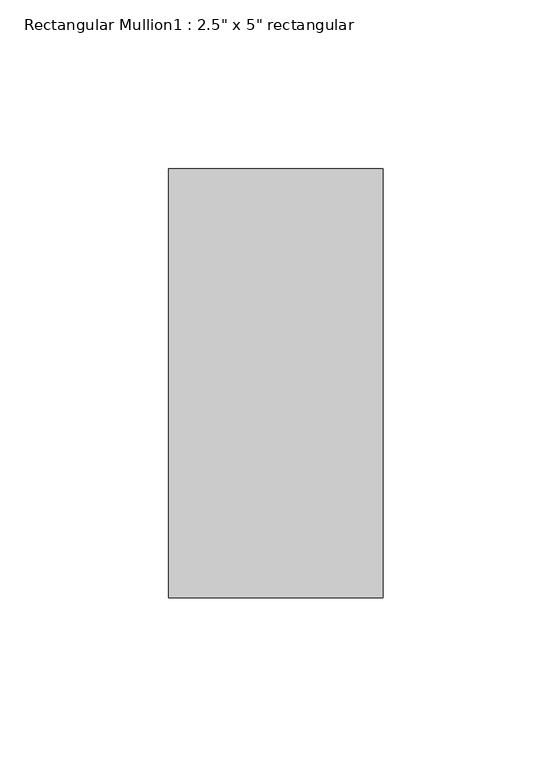
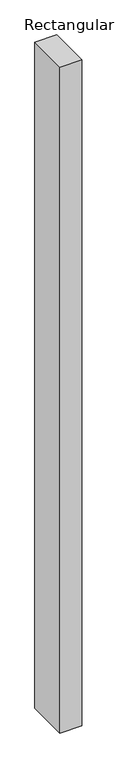
"""IFC4 building model written with IfcOpenShell, lengths in millimetres: member geometry."""

from ifc_helpers import new_model, si_unit, frame, origin, place, context, project, spatial, polyline, outline, extrude, source, transform, mapped, element, save


def member_6457a162(model_context):
    return source(origin(), model_context, "Body", "SweptSolid", [
        extrude(outline(polyline([(31.75, 63.5), (31.75, -63.5), (-31.75, -63.5), (-31.75, 63.5), (31.75, 63.5)])), frame((0.0, 0.0, -2059.94), z_axis=(0.0, 0.0, 1.0), x_axis=(1.0, 0.0, 0.0)), (0.0, 0.0, 1.0), 2059.94),
    ])


if __name__ == "__main__":
    model = new_model("IFC4")
    model_context = context("Model", 3, world=origin())
    ifc_project = project(units=[si_unit("LENGTHUNIT", "METRE", prefix="MILLI")], contexts=[model_context])
    site = spatial("IfcSite", under=ifc_project)
    building = spatial("IfcBuilding", under=site)
    placement = place(None, origin())
    member_shape = member_6457a162(model_context)
    element("IfcMember", 1, ObjectType="Rectangular Mullion1 : 2.5\" x 5\" rectangular", at=placement, inside=building, context=model_context, shape_type="MappedRepresentation", body=[
        mapped(member_shape, transform((0.0, 0.0, 0.0), x_axis=(1.0, 0.0, 0.0), y_axis=(0.0, 1.0, 0.0), z_axis=(0.0, 0.0, 1.0))),
    ])
    save(model, "model.ifc")

# Revit data of these elements
# Type "Rectangular Mullion1 : 2.5\" x 5\" rectangular"
#   built-in parameter 1007304 = 0.416667 (stored number, unit not read)
#   built-in parameter 1007301 = 0.104167 (stored number, unit not read)
#   built-in parameter 1007300 = 0.104167 (stored number, unit not read)
# Element 1 (IfcMember, "Rectangular Mullion1 : 2.5\" x 5\" rectangular")
#   Materials on its faces: "support-frame"
# Materials
#   "support-frame": class "Unassigned", colour RGB 233 233 233, transparency 0, Cost = 0
